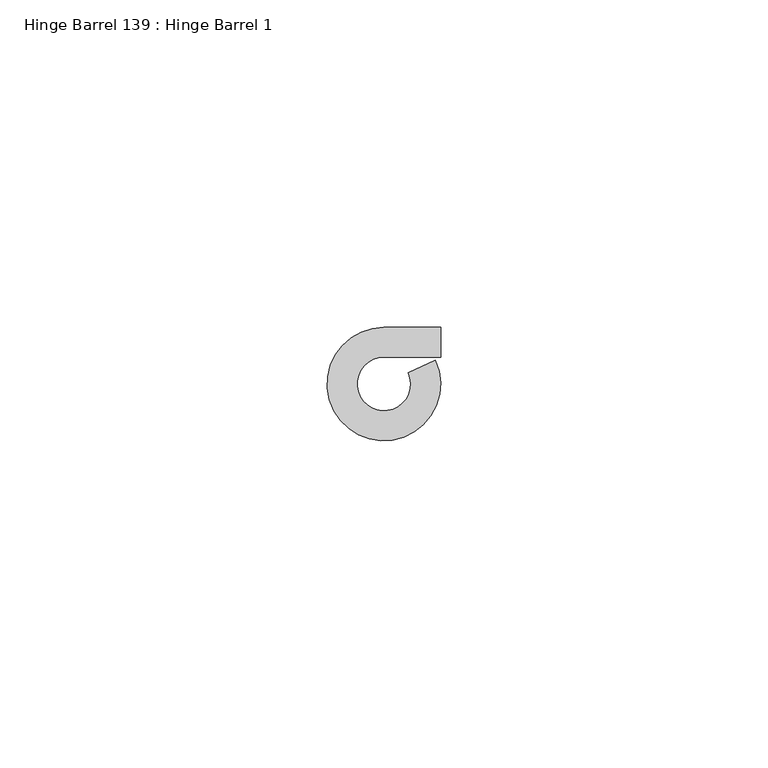
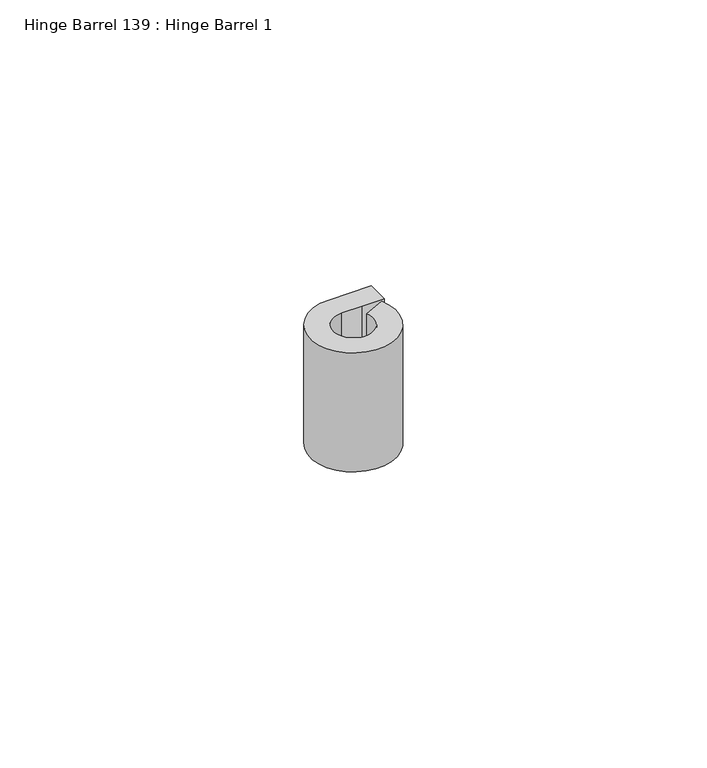
"""IFC4 building model written with IfcOpenShell, lengths in millimetres: proxy geometry, Hinge Barrel 139 : Hinge Barrel 1."""

from ifc_helpers import new_model, si_unit, point, frame, frame_2d, origin, place, context, project, spatial, polyline, circle_curve, trimmed, segment, composite_curve, outline, extrude, source, transform, mapped, element, save


def hinge_barrel_139_hinge_barrel_1_2f8cd32d(model_context):
    return source(origin(), model_context, "Body", "SweptSolid", [
        extrude(outline(composite_curve([segment(polyline([(587323.2214739, -536306.2758841), (587319.1320739, -536306.2758841)]), True, "CONTINUOUS"), segment(trimmed(circle_curve(frame_2d((587319.1320739, -536310.3652841)), 4.0894), [point((587319.1320739, -536306.2758841))], [point((587322.8436736, -536308.6485371))], True, "CARTESIAN"), True, "CONTINUOUS"), segment(polyline([(587322.8436736, -536308.6485371), (587326.986084, -536306.7325249)]), True, "CONTINUOUS"), segment(trimmed(circle_curve(frame_2d((587319.1320739, -536310.3652841)), 8.6534625), [point((587326.986084, -536306.7325249))], [point((587319.1320739, -536301.7118216))], False, "CARTESIAN"), True, "CONTINUOUS"), segment(polyline([(587319.1320739, -536301.7118216), (587327.7934739, -536301.7118216), (587327.7934739, -536306.2758841), (587323.2214739, -536306.2758841)]), True, "CONTINUOUS")], self_intersect=False)), frame((0.0, 0.0, 1123.95), z_axis=(0.0, 0.0, 1.0), x_axis=(1.0, 0.0, 0.0)), (0.0, 0.0, 1.0), 25.4),
    ])


if __name__ == "__main__":
    model = new_model("IFC4")
    model_context = context("Model", 3, world=origin())
    ifc_project = project(units=[si_unit("LENGTHUNIT", "METRE", prefix="MILLI")], contexts=[model_context])
    site = spatial("IfcSite", under=ifc_project)
    building = spatial("IfcBuilding", under=site)
    placement = place(None, origin())
    hinge_barrel_139_hinge_barrel_1_shape = hinge_barrel_139_hinge_barrel_1_2f8cd32d(model_context)
    element("IfcBuildingElementProxy", 1, Name="Hinge Barrel 139 : Hinge Barrel 1", ObjectType="Hinge Barrel 139 : Hinge Barrel 1", at=placement, inside=building, context=model_context, shape_type="MappedRepresentation", body=[
        mapped(hinge_barrel_139_hinge_barrel_1_shape, transform((0.0, 0.0, 0.0), x_axis=(1.0, 0.0, 0.0), y_axis=(0.0, 1.0, 0.0), z_axis=(0.0, 0.0, 1.0))),
    ])
    save(model, "model.ifc")

# Revit data of these elements
# Element 1 (IfcBuildingElementProxy, "Hinge Barrel 139 : Hinge Barrel 1")
#   Materials on its faces: "6\"X6\" WELD-ON STL BUTT HINGE"
# Materials
#   "6\"X6\" WELD-ON STL BUTT HINGE": class "Metal", colour RGB 189 187 185, transparency 0, Description = "Carbon steel", Cost = 0
